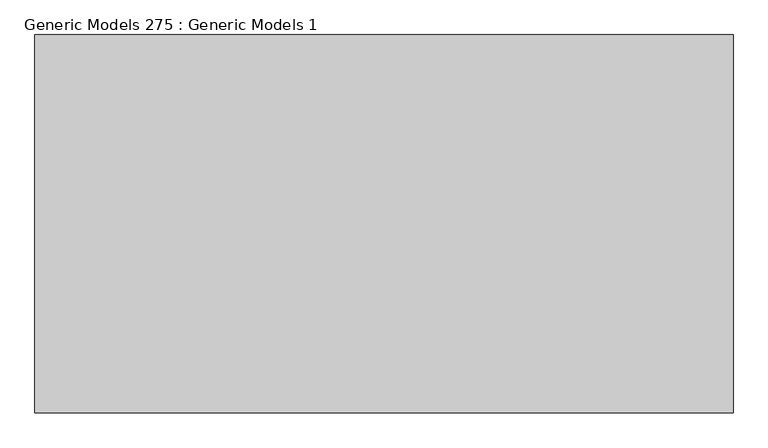
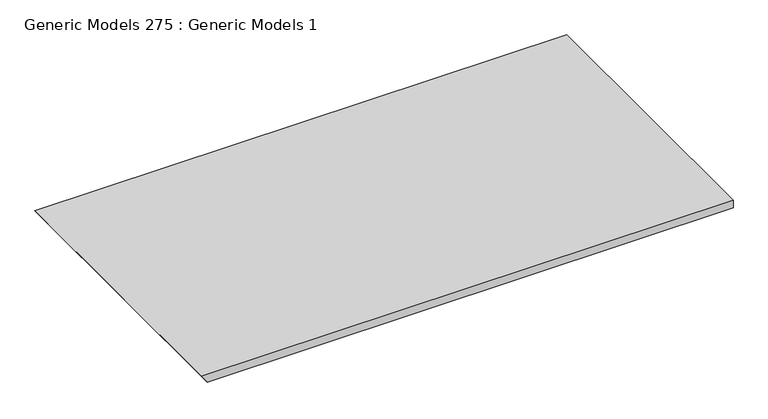
"""IFC4 building model written with IfcOpenShell, lengths in millimetres: proxy geometry, Generic Models 275 : Generic Models 1."""

from ifc_helpers import new_model, si_unit, frame, origin, place, context, project, spatial, polyline, outline, extrude, source, transform, mapped, element, save


def generic_models_275_generic_models_1_ff2c2341(model_context):
    return source(origin(), model_context, "Body", "SweptSolid", [
        extrude(outline(polyline([(126802.896, 4197.9864073), (126802.896, 2933.5263704), (126783.846, 2946.9804357), (126783.846, 4197.9864073), (126802.896, 4197.9864073)])), frame((0.0, 399.7309662, 0.0), z_axis=(0.0, 1.0, 0.0), x_axis=(0.0, 0.0, 1.0)), (0.0, 0.0, 1.0), 685.546),
    ])


if __name__ == "__main__":
    model = new_model("IFC4")
    model_context = context("Model", 3, world=origin())
    ifc_project = project(units=[si_unit("LENGTHUNIT", "METRE", prefix="MILLI")], contexts=[model_context])
    site = spatial("IfcSite", under=ifc_project)
    building = spatial("IfcBuilding", under=site)
    placement = place(None, origin())
    generic_models_275_generic_models_1_shape = generic_models_275_generic_models_1_ff2c2341(model_context)
    element("IfcBuildingElementProxy", 1, Name="Generic Models 275 : Generic Models 1", ObjectType="Generic Models 275 : Generic Models 1", at=placement, inside=building, context=model_context, shape_type="MappedRepresentation", body=[
        mapped(generic_models_275_generic_models_1_shape, transform((0.0, 0.0, 0.0), x_axis=(1.0, 0.0, 0.0), y_axis=(0.0, 1.0, 0.0), z_axis=(0.0, 0.0, 1.0))),
    ])
    save(model, "model.ifc")

# Revit data of these elements
# Element 1 (IfcBuildingElementProxy, "Generic Models 275 : Generic Models 1")
#   Materials on its faces: "_WOOD FLOORING (SPEC T.B.D.)"
# Materials
#   "_WOOD FLOORING (SPEC T.B.D.)": class "Generic", colour RGB 177 130 114, transparency 0, Cost = 0
